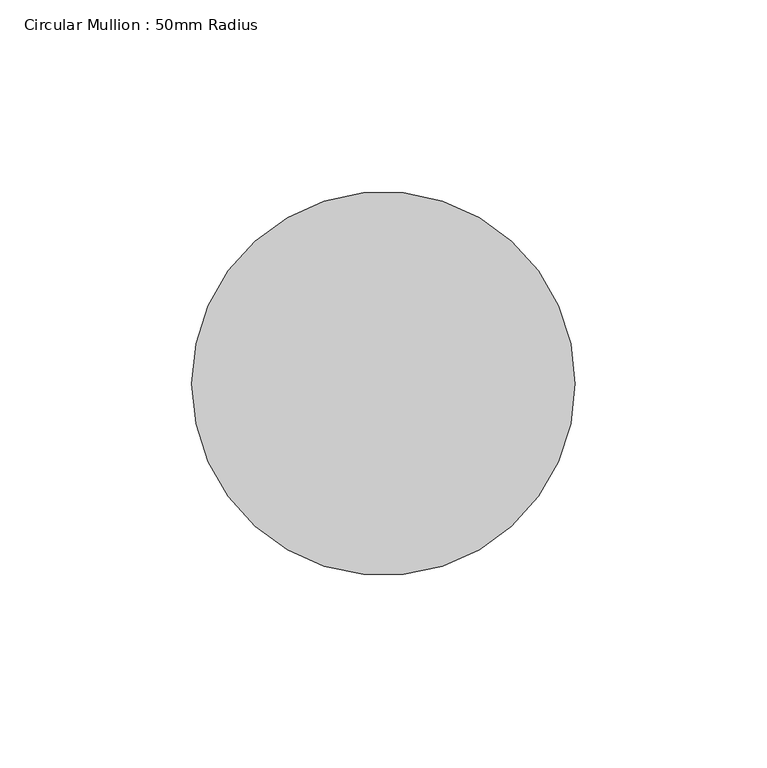
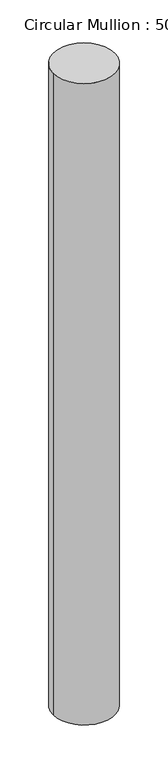
"""IFC4 building model written with IfcOpenShell, lengths in millimetres: member geometry, Circular Mullion : 50mm Radius."""

import ifcopenshell
import ifcopenshell.guid

model = None  # the IFC model being written
_history = None  # IfcOwnerHistory: only IFC2X3 demands one
_inside = {}  # id of a spatial element -> (the spatial element, [elements in it])
_under = {}  # id of a project, library or spatial element -> (it, [spatial elements below it])
_declared = {}  # id of a project -> (the project, [libraries it declares])
_typed = {}  # id of a type object -> (the type object, [elements of that type])
_made_of = {}  # id of a material, layer set ... -> (it, [elements and type objects made of it])


def new_model(schema):
    """Start an empty IFC model of exactly this schema.

    Asked for "IFC4X3", IfcOpenShell would pick the latest addendum, in which some entities
    have other attributes; the version numbers below select the first issue.
    IFC2X3 requires an IfcOwnerHistory on every rooted entity: one is made here for all.
    """
    global model, _history
    if schema == "IFC4X3":
        model = ifcopenshell.file(schema_version=(4, 3, 0, 0))
    else:
        model = ifcopenshell.file(schema=schema)
    _inside.clear()
    _under.clear()
    _declared.clear()
    _typed.clear()
    _made_of.clear()
    _history = None
    if model.schema == "IFC2X3":
        org = make("IfcOrganization", Name="unknown")
        user = make(
            "IfcPersonAndOrganization",
            ThePerson=make("IfcPerson", FamilyName="unknown"),
            TheOrganization=org,
        )
        app = make(
            "IfcApplication",
            ApplicationDeveloper=org,
            Version="unknown",
            ApplicationFullName="unknown",
            ApplicationIdentifier="unknown",
        )
        _history = make(
            "IfcOwnerHistory",
            OwningUser=user,
            OwningApplication=app,
            ChangeAction="ADDED",
            CreationDate=0,
        )
    return model


def make(cls, **values):
    """One entity of the class cls with the attributes given. An attribute that is None is left unset."""
    return model.create_entity(
        cls, **{name: value for name, value in values.items() if value is not None}
    )


def rooted(cls, **values):
    """An entity with a GlobalId (a new one), such as an element, a storey or a relation."""
    return make(cls, GlobalId=ifcopenshell.guid.new(), OwnerHistory=_history, **values)


def si_unit(unit_type, name, prefix=None):
    """IfcSIUnit, for example si_unit("LENGTHUNIT", "METRE", prefix="MILLI")."""
    return make("IfcSIUnit", UnitType=unit_type, Prefix=prefix, Name=name)


def assignment(units):
    """IfcUnitAssignment: the units of a project."""
    return None if units is None else make("IfcUnitAssignment", Units=units)


def point(xyz):
    """IfcCartesianPoint."""
    return None if xyz is None else make("IfcCartesianPoint", Coordinates=xyz)


def direction(xyz):
    """IfcDirection."""
    return None if xyz is None else make("IfcDirection", DirectionRatios=xyz)


def frame(location, z_axis=None, x_axis=None):
    """IfcAxis2Placement3D, a coordinate frame: its origin and axes. An axis left out is left unset."""
    return make(
        "IfcAxis2Placement3D",
        Location=point(location),
        Axis=direction(z_axis),
        RefDirection=direction(x_axis),
    )


def frame_2d(location, x_axis=None):
    """IfcAxis2Placement2D, a coordinate frame in the plane: its origin and x axis."""
    return make(
        "IfcAxis2Placement2D", Location=point(location), RefDirection=direction(x_axis)
    )


def origin():
    """The frame at (0, 0, 0) with its axes left unset."""
    return frame((0.0, 0.0, 0.0))


def origin_2d():
    """The frame at (0, 0) in the plane with its x axis left unset."""
    return frame_2d((0.0, 0.0))


def place(relative_to, where):
    """IfcLocalPlacement: puts the frame where relative to a parent placement (None: the world)."""
    return make(
        "IfcLocalPlacement", PlacementRelTo=relative_to, RelativePlacement=where
    )


def context(
    kind, dimensions, precision=None, world=None, true_north=None, identifier=None
):
    """IfcGeometricRepresentationContext, for example the 3D "Model" context."""
    return make(
        "IfcGeometricRepresentationContext",
        ContextIdentifier=identifier,
        ContextType=kind,
        CoordinateSpaceDimension=dimensions,
        Precision=precision,
        WorldCoordinateSystem=world,
        TrueNorth=true_north,
    )


def project(units=None, contexts=None):
    """IfcProject with its units and contexts."""
    return rooted(
        "IfcProject",
        Name="project",
        RepresentationContexts=contexts,
        UnitsInContext=assignment(units),
    )


def spatial(cls, under=None, at=None, **own):
    """A site, building, storey or space (cls), placed at a placement, below another one or the project."""
    s = rooted(cls, ObjectPlacement=at, **own)
    if under is not None:
        _under.setdefault(under.id(), (under, []))[1].append(s)
    return s


def circle_curve(where, radius):
    """IfcCircle in the frame where."""
    return make("IfcCircle", Position=where, Radius=radius)


def trimmed(basis, trim1, trim2, sense, master):
    """IfcTrimmedCurve: the piece of a basis curve between two trims."""
    return make(
        "IfcTrimmedCurve",
        BasisCurve=basis,
        Trim1=trim1,
        Trim2=trim2,
        SenseAgreement=sense,
        MasterRepresentation=master,
    )


def segment(curve, same_sense, transition):
    """IfcCompositeCurveSegment."""
    return make(
        "IfcCompositeCurveSegment",
        Transition=transition,
        SameSense=same_sense,
        ParentCurve=curve,
    )


def composite_curve(segments, self_intersect=None):
    """IfcCompositeCurve: segments joined end to end."""
    return make("IfcCompositeCurve", Segments=segments, SelfIntersect=self_intersect)


def outline(outer, holes=None, kind="AREA"):
    """IfcArbitraryClosedProfileDef: a profile drawn as a closed curve; with holes, ...WithVoids."""
    if holes is None:
        return make("IfcArbitraryClosedProfileDef", ProfileType=kind, OuterCurve=outer)
    return make(
        "IfcArbitraryProfileDefWithVoids",
        ProfileType=kind,
        OuterCurve=outer,
        InnerCurves=holes,
    )


def extrude(swept, where, along, depth):
    """IfcExtrudedAreaSolid: the profile swept, set in the frame where, extruded along a direction by depth."""
    return make(
        "IfcExtrudedAreaSolid",
        SweptArea=swept,
        Position=where,
        ExtrudedDirection=direction(along),
        Depth=depth,
    )


def shape(context_of_items, identifier, shape_type, items):
    """IfcShapeRepresentation: the items that make up one representation, for example the "Body"."""
    return make(
        "IfcShapeRepresentation",
        ContextOfItems=context_of_items,
        RepresentationIdentifier=identifier,
        RepresentationType=shape_type,
        Items=items,
    )


def source(mapping_origin, context_of_items, identifier, shape_type, items):
    """IfcRepresentationMap: a shape defined once, which mapped items show again and again."""
    return make(
        "IfcRepresentationMap",
        MappingOrigin=mapping_origin,
        MappedRepresentation=shape(context_of_items, identifier, shape_type, items),
    )


def transform(
    local_origin,
    x_axis=None,
    y_axis=None,
    z_axis=None,
    scale=None,
    scale2=None,
    scale3=None,
    uniform=True,
):
    """IfcCartesianTransformationOperator3D, or its non-uniform kind. x_axis, y_axis, z_axis: its Axis1, 2, 3."""
    if uniform:
        return make(
            "IfcCartesianTransformationOperator3D",
            Axis1=direction(x_axis),
            Axis2=direction(y_axis),
            LocalOrigin=point(local_origin),
            Scale=scale,
            Axis3=direction(z_axis),
        )
    return make(
        "IfcCartesianTransformationOperator3DnonUniform",
        Axis1=direction(x_axis),
        Axis2=direction(y_axis),
        LocalOrigin=point(local_origin),
        Scale=scale,
        Axis3=direction(z_axis),
        Scale2=scale2,
        Scale3=scale3,
    )


def mapped(mapping_source, mapping_target):
    """IfcMappedItem: shows the shape of a source again, moved by a transform."""
    return make(
        "IfcMappedItem", MappingSource=mapping_source, MappingTarget=mapping_target
    )


def made_of(thing, what):
    """Note that an element or type object is made of a material, layer set ...; save() writes the relation."""
    if what is not None:
        _made_of.setdefault(what.id(), (what, []))[1].append(thing)
    return thing


def element(
    cls,
    number,
    at=None,
    inside=None,
    cuts=None,
    type_object=None,
    material=None,
    context=None,
    identifier="Body",
    shape_type=None,
    held_by="IfcProductDefinitionShape",
    body=None,
    shapes=None,
    **own,
):
    """One element of the class cls, such as IfcWall. Its Tag is "e" and its number.

    at: its placement. inside: the storey or other place that contains it. cuts: it is an
    opening in that element (IfcRelVoidsElement). A single representation is given by context,
    identifier, shape_type and body (its items); several are given by shapes. held_by: the class
    of the entity that holds the representations. save() writes the other relations.
    """
    e = rooted(cls, Tag="e%d" % number, ObjectPlacement=at, **own)
    if body is not None:
        shapes = [shape(context, identifier, shape_type, body)]
    if shapes is not None:
        e.Representation = make(held_by, Representations=shapes)
    if inside is not None:
        _inside.setdefault(inside.id(), (inside, []))[1].append(e)
    if cuts is not None:
        rooted(
            "IfcRelVoidsElement", RelatingBuildingElement=cuts, RelatedOpeningElement=e
        )
    if type_object is not None:
        _typed.setdefault(type_object.id(), (type_object, []))[1].append(e)
    return made_of(e, material)


def aggregate(whole, parts):
    """IfcRelAggregates: a whole, such as a stair, and the parts it consists of."""
    return rooted("IfcRelAggregates", RelatingObject=whole, RelatedObjects=parts)


def save(model, path):
    """Write the relations noted so far, then the file.

    IfcRelAggregates (storeys below a building ...), IfcRelContainedInSpatialStructure (elements
    in a storey), IfcRelDefinesByType, IfcRelAssociatesMaterial and IfcRelDeclares: one each for
    every whole, place, type object, material and project.
    """
    for whole, parts in _under.values():
        aggregate(whole, parts)
    for where, things in _inside.values():
        rooted(
            "IfcRelContainedInSpatialStructure",
            RelatedElements=things,
            RelatingStructure=where,
        )
    for kind, things in _typed.values():
        rooted("IfcRelDefinesByType", RelatedObjects=things, RelatingType=kind)
    for what, things in _made_of.values():
        rooted("IfcRelAssociatesMaterial", RelatedObjects=things, RelatingMaterial=what)
    for by, libraries in _declared.values():
        rooted("IfcRelDeclares", RelatingContext=by, RelatedDefinitions=libraries)
    model.write(path)


def circular_mullion_50mm_radius_9ab308c8(model_context):
    return source(origin(), model_context, "Body", "SweptSolid", [
        extrude(outline(composite_curve([segment(trimmed(circle_curve(origin_2d(), 50.0), [point((50.0, 0.0))], [point((-50.0, 0.0))], False, "CARTESIAN"), True, "CONTINUOUS"), segment(trimmed(circle_curve(origin_2d(), 50.0), [point((-50.0, 0.0))], [point((50.0, 0.0))], False, "CARTESIAN"), True, "CONTINUOUS")], self_intersect=False)), frame((0.0, 0.0, -1104.2961794), z_axis=(0.0, 0.0, 1.0), x_axis=(1.0, 0.0, 0.0)), (0.0, 0.0, 1.0), 1104.2961794),
    ])


if __name__ == "__main__":
    model = new_model("IFC4")
    model_context = context("Model", 3, world=origin())
    ifc_project = project(units=[si_unit("LENGTHUNIT", "METRE", prefix="MILLI")], contexts=[model_context])
    site = spatial("IfcSite", under=ifc_project)
    building = spatial("IfcBuilding", under=site)
    placement = place(None, origin())
    circular_mullion_50mm_radius_shape = circular_mullion_50mm_radius_9ab308c8(model_context)
    element("IfcMember", 1, ObjectType="Circular Mullion : 50mm Radius", at=placement, inside=building, context=model_context, shape_type="MappedRepresentation", body=[
        mapped(circular_mullion_50mm_radius_shape, transform((0.0, 0.0, 0.0), x_axis=(1.0, 0.0, 0.0), y_axis=(0.0, 1.0, 0.0), z_axis=(0.0, 0.0, 1.0))),
    ])
    save(model, "model.ifc")

# Revit data of these elements
# Type "Circular Mullion : 50mm Radius"
#   built-in parameter 1007350 = 0.164042 (stored number, unit not read)
# Element 1 (IfcMember, "Circular Mullion : 50mm Radius")
#   Materials on its faces: "Aluminium"
# Materials
#   "Aluminium": class "Metal", colour RGB 247 247 247, transparency 0, Description = "Aluminium 6061", Cost = 0
